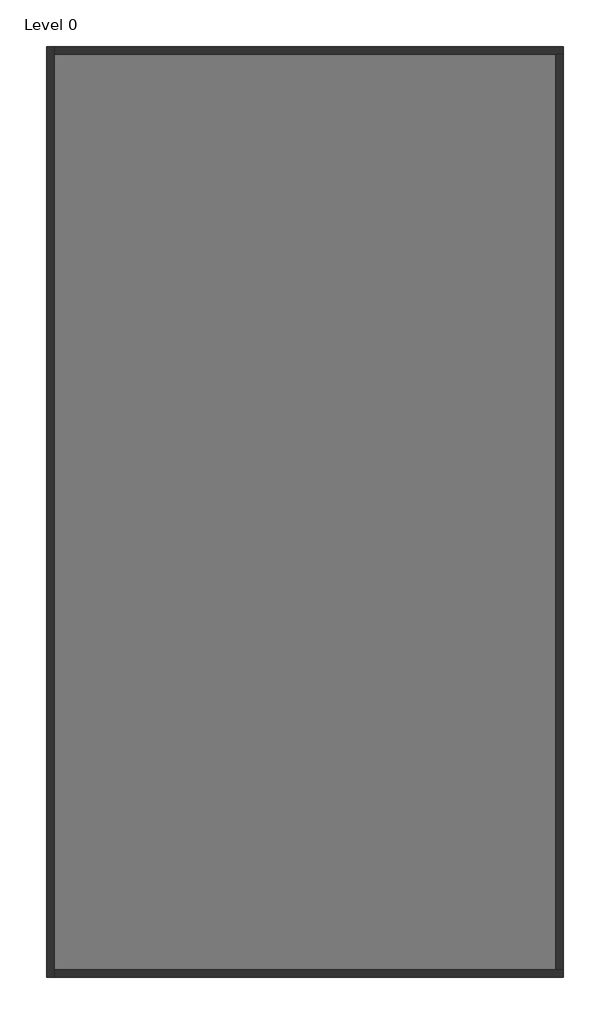
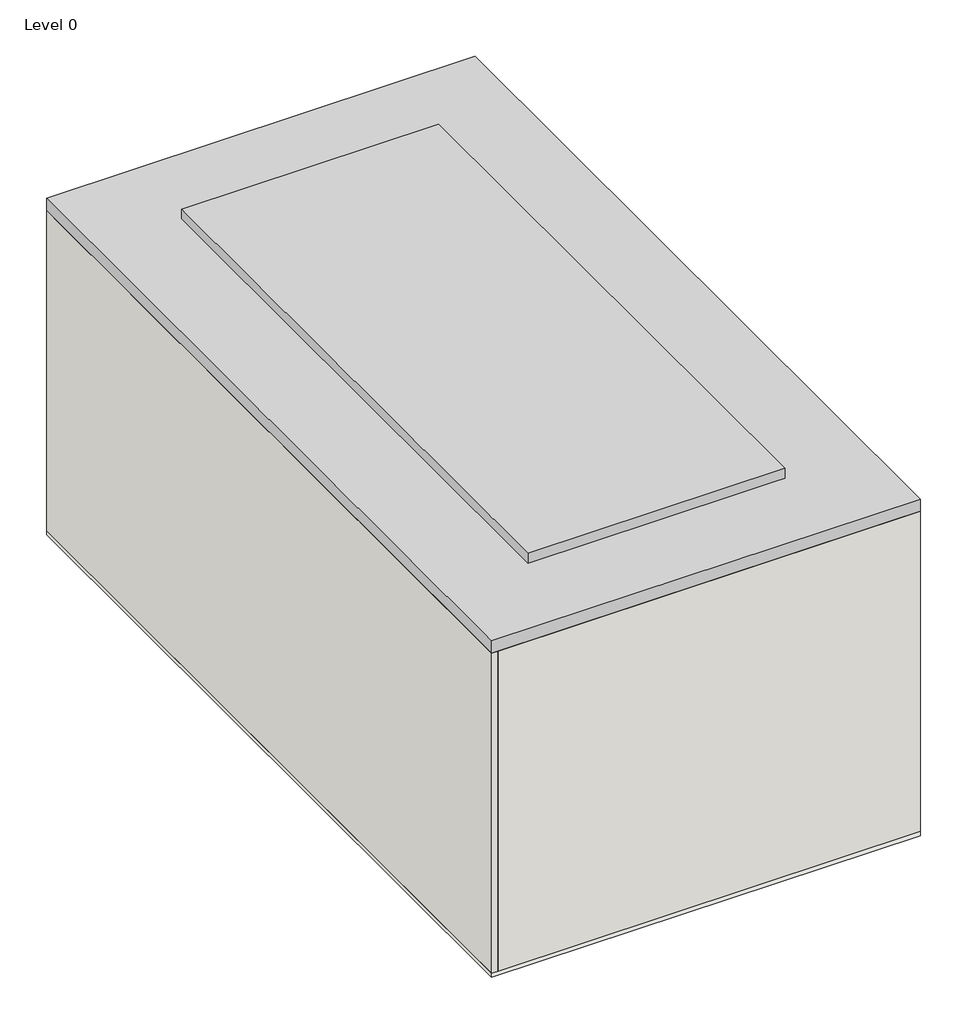
# One storey: 4 walls, 1 proxy, 1 slab.
"""IFC4 building model written with IfcOpenShell, lengths in millimetres."""

import ifcopenshell
import ifcopenshell.guid

model = None  # the IFC model being written
_history = None  # IfcOwnerHistory: only IFC2X3 demands one
_inside = {}  # id of a spatial element -> (the spatial element, [elements in it])
_under = {}  # id of a project, library or spatial element -> (it, [spatial elements below it])
_declared = {}  # id of a project -> (the project, [libraries it declares])
_typed = {}  # id of a type object -> (the type object, [elements of that type])
_made_of = {}  # id of a material, layer set ... -> (it, [elements and type objects made of it])


def new_model(schema):
    """Start an empty IFC model of exactly this schema.

    Asked for "IFC4X3", IfcOpenShell would pick the latest addendum, in which some entities
    have other attributes; the version numbers below select the first issue.
    IFC2X3 requires an IfcOwnerHistory on every rooted entity: one is made here for all.
    """
    global model, _history
    if schema == "IFC4X3":
        model = ifcopenshell.file(schema_version=(4, 3, 0, 0))
    else:
        model = ifcopenshell.file(schema=schema)
    _inside.clear()
    _under.clear()
    _declared.clear()
    _typed.clear()
    _made_of.clear()
    _history = None
    if model.schema == "IFC2X3":
        org = make("IfcOrganization", Name="unknown")
        user = make(
            "IfcPersonAndOrganization",
            ThePerson=make("IfcPerson", FamilyName="unknown"),
            TheOrganization=org,
        )
        app = make(
            "IfcApplication",
            ApplicationDeveloper=org,
            Version="unknown",
            ApplicationFullName="unknown",
            ApplicationIdentifier="unknown",
        )
        _history = make(
            "IfcOwnerHistory",
            OwningUser=user,
            OwningApplication=app,
            ChangeAction="ADDED",
            CreationDate=0,
        )
    return model


def make(cls, **values):
    """One entity of the class cls with the attributes given. An attribute that is None is left unset."""
    return model.create_entity(
        cls, **{name: value for name, value in values.items() if value is not None}
    )


def rooted(cls, **values):
    """An entity with a GlobalId (a new one), such as an element, a storey or a relation."""
    return make(cls, GlobalId=ifcopenshell.guid.new(), OwnerHistory=_history, **values)


def si_unit(unit_type, name, prefix=None):
    """IfcSIUnit, for example si_unit("LENGTHUNIT", "METRE", prefix="MILLI")."""
    return make("IfcSIUnit", UnitType=unit_type, Prefix=prefix, Name=name)


def assignment(units):
    """IfcUnitAssignment: the units of a project."""
    return None if units is None else make("IfcUnitAssignment", Units=units)


def point(xyz):
    """IfcCartesianPoint."""
    return None if xyz is None else make("IfcCartesianPoint", Coordinates=xyz)


def direction(xyz):
    """IfcDirection."""
    return None if xyz is None else make("IfcDirection", DirectionRatios=xyz)


def frame(location, z_axis=None, x_axis=None):
    """IfcAxis2Placement3D, a coordinate frame: its origin and axes. An axis left out is left unset."""
    return make(
        "IfcAxis2Placement3D",
        Location=point(location),
        Axis=direction(z_axis),
        RefDirection=direction(x_axis),
    )


def origin():
    """The frame at (0, 0, 0) with its axes left unset."""
    return frame((0.0, 0.0, 0.0))


def origin_with_axes():
    """The frame at (0, 0, 0) with the z axis (0, 0, 1) and the x axis (1, 0, 0) written out."""
    return frame((0.0, 0.0, 0.0), z_axis=(0.0, 0.0, 1.0), x_axis=(1.0, 0.0, 0.0))


def place(relative_to, where):
    """IfcLocalPlacement: puts the frame where relative to a parent placement (None: the world)."""
    return make(
        "IfcLocalPlacement", PlacementRelTo=relative_to, RelativePlacement=where
    )


def context(
    kind, dimensions, precision=None, world=None, true_north=None, identifier=None
):
    """IfcGeometricRepresentationContext, for example the 3D "Model" context."""
    return make(
        "IfcGeometricRepresentationContext",
        ContextIdentifier=identifier,
        ContextType=kind,
        CoordinateSpaceDimension=dimensions,
        Precision=precision,
        WorldCoordinateSystem=world,
        TrueNorth=true_north,
    )


def project(units=None, contexts=None):
    """IfcProject with its units and contexts."""
    return rooted(
        "IfcProject",
        Name="project",
        RepresentationContexts=contexts,
        UnitsInContext=assignment(units),
    )


def spatial(cls, under=None, at=None, **own):
    """A site, building, storey or space (cls), placed at a placement, below another one or the project."""
    s = rooted(cls, ObjectPlacement=at, **own)
    if under is not None:
        _under.setdefault(under.id(), (under, []))[1].append(s)
    return s


def polyline(points):
    """IfcPolyline through the points."""
    return make("IfcPolyline", Points=[point(p) for p in points])


def outline(outer, holes=None, kind="AREA"):
    """IfcArbitraryClosedProfileDef: a profile drawn as a closed curve; with holes, ...WithVoids."""
    if holes is None:
        return make("IfcArbitraryClosedProfileDef", ProfileType=kind, OuterCurve=outer)
    return make(
        "IfcArbitraryProfileDefWithVoids",
        ProfileType=kind,
        OuterCurve=outer,
        InnerCurves=holes,
    )


def extrude(swept, where, along, depth):
    """IfcExtrudedAreaSolid: the profile swept, set in the frame where, extruded along a direction by depth."""
    return make(
        "IfcExtrudedAreaSolid",
        SweptArea=swept,
        Position=where,
        ExtrudedDirection=direction(along),
        Depth=depth,
    )


def faces_of(points, faces, orient=None, outer=None):
    """IfcFace entities. A face is a list of loops; a loop is a list of indices into points, from 0.

    orient and outer hold one flag for each loop. By default every Orientation is true, the
    first loop of a face is its IfcFaceOuterBound and the others are IfcFaceBound.
    """
    made = []
    for i, loops in enumerate(faces):
        bounds = []
        for j, loop in enumerate(loops):
            is_outer = j == 0 if outer is None else outer[i][j]
            bounds.append(
                make(
                    "IfcFaceOuterBound" if is_outer else "IfcFaceBound",
                    Bound=make("IfcPolyLoop", Polygon=[points[k] for k in loop]),
                    Orientation=True if orient is None else orient[i][j],
                )
            )
        made.append(make("IfcFace", Bounds=bounds))
    return made


def faceted_brep(points, faces, orient=None, outer=None, voids=None):
    """IfcFacetedBrep: a solid bounded by flat faces; with voids (closed shells), ...WithVoids."""
    shared = [point(p) for p in points]
    hull = make("IfcClosedShell", CfsFaces=faces_of(shared, faces, orient, outer))
    if voids is None:
        return make("IfcFacetedBrep", Outer=hull)
    return make(
        "IfcFacetedBrepWithVoids",
        Outer=hull,
        Voids=[
            make(cls, CfsFaces=faces_of(shared, fs, o, b)) for cls, fs, o, b in voids
        ],
    )


def shape(context_of_items, identifier, shape_type, items):
    """IfcShapeRepresentation: the items that make up one representation, for example the "Body"."""
    return make(
        "IfcShapeRepresentation",
        ContextOfItems=context_of_items,
        RepresentationIdentifier=identifier,
        RepresentationType=shape_type,
        Items=items,
    )


def made_of(thing, what):
    """Note that an element or type object is made of a material, layer set ...; save() writes the relation."""
    if what is not None:
        _made_of.setdefault(what.id(), (what, []))[1].append(thing)
    return thing


def element(
    cls,
    number,
    at=None,
    inside=None,
    cuts=None,
    type_object=None,
    material=None,
    context=None,
    identifier="Body",
    shape_type=None,
    held_by="IfcProductDefinitionShape",
    body=None,
    shapes=None,
    **own,
):
    """One element of the class cls, such as IfcWall. Its Tag is "e" and its number.

    at: its placement. inside: the storey or other place that contains it. cuts: it is an
    opening in that element (IfcRelVoidsElement). A single representation is given by context,
    identifier, shape_type and body (its items); several are given by shapes. held_by: the class
    of the entity that holds the representations. save() writes the other relations.
    """
    e = rooted(cls, Tag="e%d" % number, ObjectPlacement=at, **own)
    if body is not None:
        shapes = [shape(context, identifier, shape_type, body)]
    if shapes is not None:
        e.Representation = make(held_by, Representations=shapes)
    if inside is not None:
        _inside.setdefault(inside.id(), (inside, []))[1].append(e)
    if cuts is not None:
        rooted(
            "IfcRelVoidsElement", RelatingBuildingElement=cuts, RelatedOpeningElement=e
        )
    if type_object is not None:
        _typed.setdefault(type_object.id(), (type_object, []))[1].append(e)
    return made_of(e, material)


def aggregate(whole, parts):
    """IfcRelAggregates: a whole, such as a stair, and the parts it consists of."""
    return rooted("IfcRelAggregates", RelatingObject=whole, RelatedObjects=parts)


def save(model, path):
    """Write the relations noted so far, then the file.

    IfcRelAggregates (storeys below a building ...), IfcRelContainedInSpatialStructure (elements
    in a storey), IfcRelDefinesByType, IfcRelAssociatesMaterial and IfcRelDeclares: one each for
    every whole, place, type object, material and project.
    """
    for whole, parts in _under.values():
        aggregate(whole, parts)
    for where, things in _inside.values():
        rooted(
            "IfcRelContainedInSpatialStructure",
            RelatedElements=things,
            RelatingStructure=where,
        )
    for kind, things in _typed.values():
        rooted("IfcRelDefinesByType", RelatedObjects=things, RelatingType=kind)
    for what, things in _made_of.values():
        rooted("IfcRelAssociatesMaterial", RelatedObjects=things, RelatingMaterial=what)
    for by, libraries in _declared.values():
        rooted("IfcRelDeclares", RelatingContext=by, RelatedDefinitions=libraries)
    model.write(path)


model = new_model("IFC4")

# Units and contexts
model_context = context("Model", 3, world=origin())
ifc_project = project(units=[si_unit("LENGTHUNIT", "METRE", prefix="MILLI")], contexts=[model_context])

# Site, building, storey
site = spatial("IfcSite", under=ifc_project)
building = spatial("IfcBuilding", under=site)
storey = spatial("IfcBuildingStorey", under=building, Name="Level 0", Elevation=100.0)

# Proxy
placement = place(None, origin())
element("IfcBuildingElementProxy", 1, Name="LowUrbanDensityBuilding : LowUrbanDensityBuilding", ObjectType="LowUrbanDensityBuilding : LowUrbanDensityBuilding", at=placement, inside=storey, context=model_context, shape_type="SweptSolid", body=[
    extrude(outline(polyline([(7325.2659446, 3676.2074539), (7325.2659446, -14323.7925461), (-2674.7340554, -14323.7925461), (-2674.7340554, 3676.2074539), (7325.2659446, 3676.2074539)])), origin_with_axes(), (0.0, 0.0, 1.0), 8300.0),
    extrude(outline(polyline([(5325.2659446, 1676.2074539), (5325.2659446, -12323.7925461), (-674.7340554, -12323.7925461), (-674.7340554, 1676.2074539), (5325.2659446, 1676.2074539)])), frame((0.0, 0.0, 8300.0), z_axis=(0.0, 0.0, 1.0), x_axis=(1.0, 0.0, 0.0)), (0.0, 0.0, 1.0), 245.0),
])

# Slab
element("IfcSlab", 2, ObjectType="Floor-Concrete_100Con", at=placement, inside=storey, context=model_context, shape_type="SweptSolid", body=[
    extrude(outline(polyline([(7325.2659446, 3676.2074539), (7325.2659446, -14323.7925461), (-2674.7340554, -14323.7925461), (-2674.7340554, 3676.2074539), (7325.2659446, 3676.2074539)])), origin_with_axes(), (0.0, 0.0, 1.0), 100.0),
])

# Walls
element("IfcWall", 3, ObjectType="Wall-Ext_25Rdr-100Blk-19P", at=placement, inside=storey, context=model_context, shape_type="Brep", body=[
    faceted_brep([(-2674.7340554, 3676.2074539, 100.0), (-2674.7340554, -14323.7925461, 100.0), (-2674.7340554, -14323.7925461, 8000.0), (-2674.7340554, 3676.2074539, 8000.0), (-2530.4340554, 3676.2074539, 100.0), (-2530.4340554, 3676.2074539, 8000.0), (-2530.4340554, 3531.9074539, 8000.0), (-2530.4340554, -14179.4925461, 8000.0), (-2530.4340554, -14323.7925461, 8000.0), (-2530.4340554, -14323.7925461, 100.0), (-2530.4340554, -14179.4925461, 100.0), (-2530.4340554, 3531.9074539, 100.0)], [[[0, 1, 2, 3]], [[4, 5, 6, 7, 8, 9, 10, 11]], [[1, 0, 4, 11, 10, 9]], [[3, 2, 8, 7, 6, 5]], [[2, 1, 9, 8]], [[0, 3, 5, 4]]]),
])
element("IfcWall", 4, ObjectType="Wall-Ext_25Rdr-100Blk-19P", at=placement, inside=storey, context=model_context, shape_type="Brep", body=[
    faceted_brep([(-2530.4340554, -14323.7925461, 100.0), (7325.2659446, -14323.7925461, 100.0), (7325.2659446, -14323.7925461, 8000.0), (-2530.4340554, -14323.7925461, 8000.0), (-2530.4340554, -14179.4925461, 100.0), (-2530.4340554, -14179.4925461, 8000.0), (7180.9659446, -14179.4925461, 8000.0), (7325.2659446, -14179.4925461, 8000.0), (7325.2659446, -14179.4925461, 100.0), (7180.9659446, -14179.4925461, 100.0)], [[[0, 1, 2, 3]], [[4, 5, 6, 7, 8, 9]], [[1, 0, 4, 9, 8]], [[3, 2, 7, 6, 5]], [[0, 3, 5, 4]], [[2, 1, 8, 7]]]),
])
element("IfcWall", 5, ObjectType="Wall-Ext_25Rdr-100Blk-19P", at=placement, inside=storey, context=model_context, shape_type="Brep", body=[
    faceted_brep([(7325.2659446, 3676.2074539, 100.0), (-2530.4340554, 3676.2074539, 100.0), (-2530.4340554, 3676.2074539, 8000.0), (7325.2659446, 3676.2074539, 8000.0), (7325.2659446, 3531.9074539, 100.0), (7325.2659446, 3531.9074539, 8000.0), (7180.9659446, 3531.9074539, 8000.0), (-2530.4340554, 3531.9074539, 8000.0), (-2530.4340554, 3531.9074539, 100.0), (7180.9659446, 3531.9074539, 100.0)], [[[0, 1, 2, 3]], [[4, 5, 6, 7, 8, 9]], [[1, 0, 4, 9, 8]], [[3, 2, 7, 6, 5]], [[2, 1, 8, 7]], [[0, 3, 5, 4]]]),
])
element("IfcWall", 6, ObjectType="Wall-Ext_25Rdr-100Blk-19P", at=placement, inside=storey, context=model_context, shape_type="SweptSolid", body=[
    extrude(outline(polyline([(7325.2659446, 3531.9074539), (7325.2659446, -14179.4925461), (7180.9659446, -14179.4925461), (7180.9659446, 3531.9074539), (7325.2659446, 3531.9074539)])), frame((0.0, 0.0, 100.0), z_axis=(0.0, 0.0, 1.0), x_axis=(1.0, 0.0, 0.0)), (0.0, 0.0, 1.0), 7900.0),
])

save(model, "model.ifc")

# Revit data of these elements
# Project information
#   Project Issue Date = "Issue Date"
#   Project Status = "Project Status"
#   Client Name = "Owner"
#   Project Address = "Enter address here"
#   Project Name = "Project Name"
#   Project Number = "Project Number"
# Type "Floor-Concrete_100Con"
#   Keynote = "E60/130"
#   Function = 0
#   Layers, outside or top first: 100 mm "Concrete" (function 1)
# Type "Wall-Ext_25Rdr-100Blk-19P"
#   Keynote = "F10"
#   Layers, outside or top first: 25.3 mm "Render, Beige, Smooth" (function 5); 100 mm "Concrete Masonry Units _Low Density" (function 1); 19 mm "Plaster" (function 5)
# Element 1 (IfcBuildingElementProxy, "LowUrbanDensityBuilding : LowUrbanDensityBuilding")
#   Phase Created = New Construction
#   Materials on its faces: "Default Form"
# Element 2 (IfcSlab, "Floor-Concrete_100Con")
#   Height Offset From Level = 0 mm
#   Phase Created = New Construction
#   Materials on its faces: "Concrete"
# Element 3 (IfcWall, "Wall-Ext_25Rdr-100Blk-19P")
#   Top Offset = 0 mm
#   Base Offset = 0 mm
#   wall height = 7900 mm
#   Phase Created = New Construction
#   Base Constraint = Level 0
#   Top Constraint = Level 2
#   Materials on its faces: "Render, Beige, Smooth", "Default Wall", "Plaster"
# Elements 4, 5, 6 (IfcWall, "Wall-Ext_25Rdr-100Blk-19P")
#   Top Offset = 0 mm
#   Base Offset = 0 mm
#   wall height = 7900 mm
#   Phase Created = New Construction
#   Base Constraint = Level 0
#   Top Constraint = Level 2
#   Materials on its faces: "Default Wall", "Render, Beige, Smooth", "Plaster"
# Materials
#   "Concrete": class "Concrete", colour RGB 120 120 120, transparency 0, Description = "Portland Cement Concrete", Cost = 0
#   "Render, Beige, Smooth": class "Generic", colour RGB 213 198 180, transparency 0, Description = "physical material", Cost = 0
#   "Concrete Masonry Units _Low Density": class "Masonry", colour RGB 181 181 181, transparency 0, Description = "Concrete masonry units", Cost = 0
#   "Plaster": class "Generic", colour RGB 249 249 249, transparency 0, Description = "Plaster", Cost = 0
#   "Default Form": class "Generic", colour RGB 185 189 196, transparency 0.5, Cost = 0
#   "Default Wall": class "Miscellaneous", colour RGB 128 128 128, transparency 0, Comments = "Rendering appearance not upgraded Rendering appearance not upgraded ", Cost = 0
